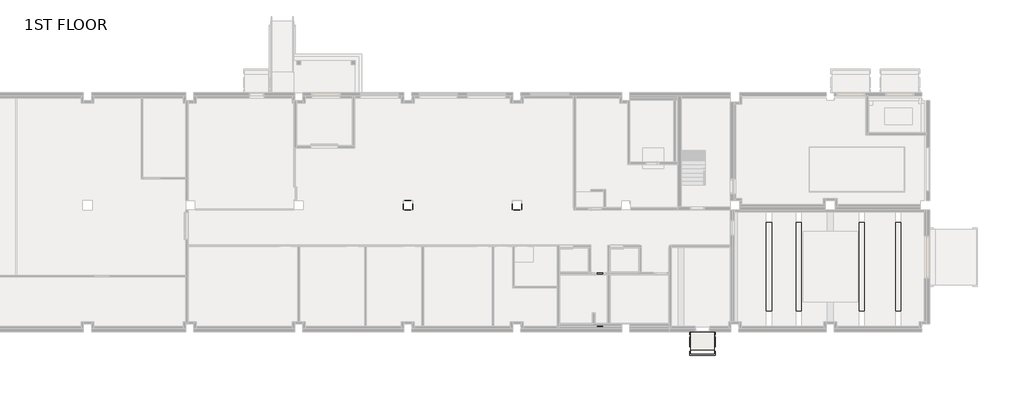
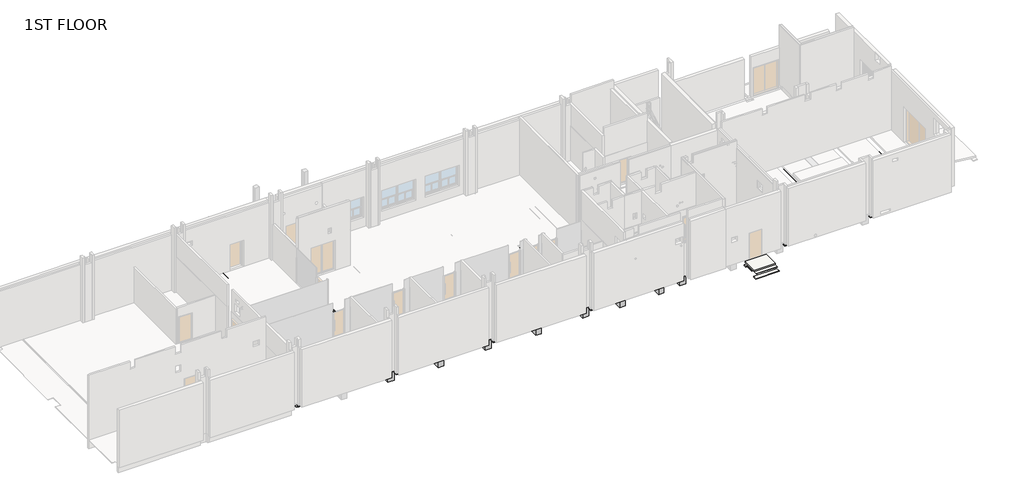
# One storey, part 9 of 15: 19 beams, 7 slabs.
"""IFC4 building model written with IfcOpenShell, lengths in millimetres."""

from ifc_helpers import new_model, si_unit, frame, origin, place, context, project, spatial, polyline, outline, extrude, faceted_brep, element, save

model = new_model("IFC4")

# Units and contexts
model_context = context("Model", 3, world=origin())
ifc_project = project(units=[si_unit("LENGTHUNIT", "METRE", prefix="MILLI")], contexts=[model_context])

# Site, building, storey
site = spatial("IfcSite", under=ifc_project)
building = spatial("IfcBuilding", under=site)
storey = spatial("IfcBuildingStorey", under=building, Name="1ST FLOOR", Elevation=4800.0)

# Beams
placement = place(None, origin())
element("IfcBeam", 1, ObjectType="RC Beam_Rectangular : H_SB_AR S16_TG-UG_500x800_1G2", at=placement, inside=storey, context=model_context, shape_type="Brep", body=[
    faceted_brep([(22650.0, -8350.0, 4800.0), (22650.0, -7850.0, 4800.0), (19225.0, -7850.0, 4800.0), (18775.0, -7850.0, 4800.0), (15400.0000001, -7850.0, 4800.0), (15400.0000001, -8350.0, 4800.0), (18775.0, -8350.0, 4800.0), (19225.0, -8350.0, 4800.0), (22650.0, -7850.0, 4000.0), (19225.0, -7850.0, 4000.0), (18775.0, -7850.0, 4000.0), (15400.0000001, -7850.0, 4000.0), (15400.0000001, -7850.0, 4650.0), (22650.0, -7850.0, 4650.0), (22650.0, -8350.0, 4000.0), (19225.0, -8350.0, 4000.0), (18775.0, -8350.0, 4000.0), (15400.0000001, -8350.0, 4000.0), (22650.0, -8350.0, 4650.0), (15400.0000001, -8350.0, 4650.0)], [[[0, 1, 2, 3, 4, 5, 6, 7]], [[8, 9, 10, 11, 12, 4, 3, 2, 1, 13]], [[11, 10, 9, 8, 14, 15, 16, 17]], [[17, 16, 15, 14, 18, 0, 7, 6, 5, 19]], [[14, 8, 13, 1, 0, 18]], [[5, 4, 12, 11, 17, 19]]]),
])
element("IfcBeam", 2, ObjectType="RC Beam_Rectangular : H_SB_AR S16_TG-UG_500x800_1G2", at=placement, inside=storey, context=model_context, shape_type="Brep", body=[
    faceted_brep([(23350.0, -7850.0, 4800.0), (23350.0, -8350.0, 4800.0), (26775.0, -8350.0, 4800.0), (27225.0, -8350.0, 4800.0), (30650.0, -8350.0, 4800.0), (30650.0, -7850.0, 4800.0), (27225.0, -7850.0, 4800.0), (26775.0, -7850.0, 4800.0), (23350.0, -8350.0, 4000.0), (26775.0, -8350.0, 4000.0), (27225.0, -8350.0, 4000.0), (30650.0, -8350.0, 4000.0), (30650.0, -8350.0, 4650.0), (23350.0, -8350.0, 4650.0), (23350.0, -7850.0, 4000.0), (26775.0, -7850.0, 4000.0), (27225.0, -7850.0, 4000.0), (30650.0, -7850.0, 4000.0), (23350.0, -7850.0, 4650.0), (30650.0, -7850.0, 4650.0)], [[[0, 1, 2, 3, 4, 5, 6, 7]], [[8, 9, 10, 11, 12, 4, 3, 2, 1, 13]], [[11, 10, 9, 8, 14, 15, 16, 17]], [[17, 16, 15, 14, 18, 0, 7, 6, 5, 19]], [[14, 8, 13, 1, 0, 18]], [[5, 4, 12, 11, 17, 19]]]),
])
element("IfcBeam", 3, ObjectType="RC Beam_Rectangular : H_SB_AR S16_TG-UG_500x800_1G2", at=placement, inside=storey, context=model_context, shape_type="Brep", body=[
    faceted_brep([(31350.0, -7850.0, 4800.0), (31350.0, -8350.0, 4800.0), (34775.0, -8350.0, 4800.0), (35225.0, -8350.0, 4800.0), (38650.0, -8350.0, 4800.0), (38650.0, -7850.0, 4800.0), (35225.0, -7850.0, 4800.0), (34775.0, -7850.0, 4800.0), (31350.0, -8350.0, 4000.0), (34775.0, -8350.0, 4000.0), (35225.0, -8350.0, 4000.0), (38650.0, -8350.0, 4000.0), (38650.0, -8350.0, 4650.0), (31350.0, -8350.0, 4650.0), (31350.0, -7850.0, 4000.0), (34775.0, -7850.0, 4000.0), (35225.0, -7850.0, 4000.0), (38650.0, -7850.0, 4000.0), (31350.0, -7850.0, 4650.0), (38650.0, -7850.0, 4650.0)], [[[0, 1, 2, 3, 4, 5, 6, 7]], [[8, 9, 10, 11, 12, 4, 3, 2, 1, 13]], [[11, 10, 9, 8, 14, 15, 16, 17]], [[17, 16, 15, 14, 18, 0, 7, 6, 5, 19]], [[14, 8, 13, 1, 0, 18]], [[5, 4, 12, 11, 17, 19]]]),
])
element("IfcBeam", 4, ObjectType="RC Beam_Rectangular : H_SB_AR S16_TG-UG_500x800_1G2", at=placement, inside=storey, context=model_context, shape_type="Brep", body=[
    faceted_brep([(39350.0, -7850.0, 4800.0), (39350.0, -8350.0, 4800.0), (41675.0, -8350.0, 4800.0), (42125.0, -8350.0, 4800.0), (44875.0, -8350.0, 4800.0), (45325.0, -8350.0, 4800.0), (46650.0, -8350.0, 4800.0), (46650.0, -7850.0, 4800.0), (45325.0, -7850.0, 4800.0), (44875.0, -7850.0, 4800.0), (42125.0, -7850.0, 4800.0), (41675.0, -7850.0, 4800.0), (39350.0, -8350.0, 4000.0), (41675.0, -8350.0, 4000.0), (42125.0, -8350.0, 4000.0), (44875.0, -8350.0, 4000.0), (45325.0, -8350.0, 4000.0), (46650.0, -8350.0, 4000.0), (46650.0, -8350.0, 4650.0), (39350.0, -8350.0, 4650.0), (39350.0, -7850.0, 4000.0), (41675.0, -7850.0, 4000.0), (42125.0, -7850.0, 4000.0), (44875.0, -7850.0, 4000.0), (45325.0, -7850.0, 4000.0), (46650.0, -7850.0, 4000.0), (39350.0, -7850.0, 4650.0), (46650.0, -7850.0, 4650.0)], [[[0, 1, 2, 3, 4, 5, 6, 7, 8, 9, 10, 11]], [[12, 13, 14, 15, 16, 17, 18, 6, 5, 4, 3, 2, 1, 19]], [[17, 16, 15, 14, 13, 12, 20, 21, 22, 23, 24, 25]], [[25, 24, 23, 22, 21, 20, 26, 0, 11, 10, 9, 8, 7, 27]], [[20, 12, 19, 1, 0, 26]], [[7, 6, 18, 17, 25, 27]]]),
])
element("IfcBeam", 5, ObjectType="RC Beam_Rectangular : H_SB_AR S16_TG-UG_500x800_1G1", at=placement, inside=storey, context=model_context, shape_type="Brep", body=[
    faceted_brep([(22700.0, -300.0, 4800.0), (22700.0, -7650.0, 4800.0), (23200.0, -7650.0, 4800.0), (23200.0, -300.0, 4800.0), (23200.0, -7650.0, 4650.0), (23200.0, -7650.0, 4000.0), (23200.0, -300.0, 4000.0), (23200.0, -300.0, 4650.0), (22700.0, -7650.0, 4000.0), (22700.0, -300.0, 4000.0), (22700.0, -300.0, 4650.0), (22700.0, -7650.0, 4650.0)], [[[0, 1, 2, 3]], [[3, 2, 4, 5, 6, 7]], [[6, 5, 8, 9]], [[1, 0, 10, 9, 8, 11]], [[8, 5, 4, 2, 1, 11]], [[0, 3, 7, 6, 9, 10]]]),
])
element("IfcBeam", 6, ObjectType="RC Beam_Rectangular : H_SB_AR S16_TG-UG_450x800_1B1", at=placement, inside=storey, context=model_context, shape_type="Brep", body=[
    faceted_brep([(19225.0, -100.0, 4800.0), (18775.0, -100.0, 4800.0), (18775.0, -7850.0, 4800.0), (19225.0, -7850.0, 4800.0), (19225.0, -7850.0, 4650.0), (19225.0, -7850.0, 4000.0), (19225.0, -100.0, 4000.0), (19225.0, -100.0, 4650.0), (18775.0, -100.0, 4000.0), (18775.0, -7850.0, 4000.0), (18775.0, -100.0, 4650.0), (18775.0, -7850.0, 4650.0)], [[[0, 1, 2, 3]], [[0, 3, 4, 5, 6, 7]], [[8, 6, 5, 9]], [[2, 1, 10, 8, 9, 11]], [[1, 0, 7, 6, 8, 10]], [[3, 2, 11, 9, 5, 4]]]),
])
element("IfcBeam", 7, ObjectType="RC Beam_Rectangular : H_SB_AR S16_TG-UG_500x800_1G1", at=placement, inside=storey, context=model_context, shape_type="Brep", body=[
    faceted_brep([(30750.0, -300.0, 4800.0), (30750.0, -7650.0, 4800.0), (31250.0, -7650.0, 4800.0), (31250.0, -300.0, 4800.0), (31250.0, -7650.0, 4650.0), (31250.0, -7650.0, 4000.0), (31250.0, -300.0, 4000.0), (31250.0, -300.0, 4650.0), (30750.0, -7650.0, 4000.0), (30750.0, -300.0, 4000.0), (30750.0, -300.0, 4650.0), (30750.0, -7650.0, 4650.0)], [[[0, 1, 2, 3]], [[3, 2, 4, 5, 6, 7]], [[6, 5, 8, 9]], [[1, 0, 10, 9, 8, 11]], [[8, 5, 4, 2, 1, 11]], [[0, 3, 7, 6, 9, 10]]]),
])
element("IfcBeam", 8, ObjectType="RC Beam_Rectangular : H_SB_AR S16_TG-UG_450x800_1B1", at=placement, inside=storey, context=model_context, shape_type="Brep", body=[
    faceted_brep([(27225.0, -100.0, 4800.0), (26775.0, -100.0, 4800.0), (26775.0, -7850.0, 4800.0), (27225.0, -7850.0, 4800.0), (27225.0, -7850.0, 4650.0), (27225.0, -7850.0, 4000.0), (27225.0, -100.0, 4000.0), (27225.0, -100.0, 4650.0), (26775.0, -100.0, 4000.0), (26775.0, -7850.0, 4000.0), (26775.0, -100.0, 4650.0), (26775.0, -7850.0, 4650.0)], [[[0, 1, 2, 3]], [[0, 3, 4, 5, 6, 7]], [[8, 6, 5, 9]], [[2, 1, 10, 8, 9, 11]], [[1, 0, 7, 6, 8, 10]], [[3, 2, 11, 9, 5, 4]]]),
])
element("IfcBeam", 9, ObjectType="RC Beam_Rectangular : H_SB_AR S16_TG-UG_450x800_1B1", at=placement, inside=storey, context=model_context, shape_type="Brep", body=[
    faceted_brep([(35225.0, -100.0, 4800.0), (34775.0, -100.0, 4800.0), (34775.0, -7850.0, 4800.0), (35225.0, -7850.0, 4800.0), (35225.0, -7850.0, 4650.0), (35225.0, -7850.0, 4000.0), (35225.0, -100.0, 4000.0), (35225.0, -100.0, 4650.0), (34775.0, -100.0, 4000.0), (34775.0, -7850.0, 4000.0), (34775.0, -100.0, 4650.0), (34775.0, -7850.0, 4650.0)], [[[0, 1, 2, 3]], [[0, 3, 4, 5, 6, 7]], [[8, 6, 5, 9]], [[2, 1, 10, 8, 9, 11]], [[1, 0, 7, 6, 8, 10]], [[3, 2, 11, 9, 5, 4]]]),
])
element("IfcBeam", 10, ObjectType="RC Beam_Rectangular : H_SB_AR S16_TG-UG_500x800_1G1", at=placement, inside=storey, context=model_context, shape_type="Brep", body=[
    faceted_brep([(22750.0, -8350.0, 4800.0), (22750.0, -16700.0, 4800.0), (23250.0, -16700.0, 4800.0), (23250.0, -8350.0, 4800.0), (23250.0, -16700.0, 4650.0), (23250.0, -16700.0, 4000.0), (23250.0, -8350.0, 4000.0), (23250.0, -8350.0, 4650.0), (22750.0, -16700.0, 4000.0), (22750.0, -8350.0, 4000.0), (22750.0, -8350.0, 4650.0), (22750.0, -16700.0, 4650.0)], [[[0, 1, 2, 3]], [[3, 2, 4, 5, 6, 7]], [[6, 5, 8, 9]], [[1, 0, 10, 9, 8, 11]], [[0, 3, 7, 6, 9, 10]], [[8, 5, 4, 2, 1, 11]]]),
])
element("IfcBeam", 11, ObjectType="RC Beam_Rectangular : H_SB_AR S16_TG-UG_500x800_1G1", at=placement, inside=storey, context=model_context, shape_type="Brep", body=[
    faceted_brep([(30750.0, -8350.0, 4800.0), (30750.0, -16700.0, 4800.0), (31250.0, -16700.0, 4800.0), (31250.0, -8350.0, 4800.0), (31250.0, -16700.0, 4650.0), (31250.0, -16700.0, 4000.0), (31250.0, -8350.0, 4000.0), (31250.0, -8350.0, 4650.0), (30750.0, -16700.0, 4000.0), (30750.0, -8350.0, 4000.0), (30750.0, -8350.0, 4650.0), (30750.0, -16700.0, 4650.0)], [[[0, 1, 2, 3]], [[3, 2, 4, 5, 6, 7]], [[6, 5, 8, 9]], [[1, 0, 10, 9, 8, 11]], [[0, 3, 7, 6, 9, 10]], [[8, 5, 4, 2, 1, 11]]]),
])
element("IfcBeam", 12, ObjectType="RC Beam_Rectangular : H_SB_AR S16_TG-UG_500x800_1G1", at=placement, inside=storey, context=model_context, shape_type="Brep", body=[
    faceted_brep([(38750.0000001, -8350.0, 4800.0), (38750.0000001, -16700.0, 4800.0), (39250.0000001, -16700.0, 4800.0), (39250.0000001, -8350.0, 4800.0), (39250.0000001, -16700.0, 4650.0), (39250.0000001, -16700.0, 4000.0), (39250.0000001, -8350.0, 4000.0), (39250.0000001, -8350.0, 4650.0), (38750.0000001, -16700.0, 4000.0), (38750.0000001, -8350.0, 4000.0), (38750.0000001, -8350.0, 4650.0), (38750.0000001, -16700.0, 4650.0)], [[[0, 1, 2, 3]], [[3, 2, 4, 5, 6, 7]], [[6, 5, 8, 9]], [[1, 0, 10, 9, 8, 11]], [[0, 3, 7, 6, 9, 10]], [[8, 5, 4, 2, 1, 11]]]),
])
element("IfcBeam", 13, ObjectType="RC Beam_Rectangular : H_SB_AR S16_TG-UG_450x800_1B1A", at=placement, inside=storey, context=model_context, shape_type="Brep", body=[
    faceted_brep([(26775.0, -16900.0, 4800.0), (27225.0, -16900.0, 4800.0), (27225.0, -8350.0, 4800.0), (26775.0, -8350.0, 4800.0), (27225.0, -16900.0, 4650.0), (27225.0, -16900.0, 4000.0), (27225.0, -8350.0, 4000.0), (27225.0, -8350.0, 4650.0), (26775.0, -16900.0, 4000.0), (26775.0, -8350.0, 4000.0), (26775.0, -8350.0, 4650.0), (26775.0, -16900.0, 4650.0)], [[[0, 1, 2, 3]], [[2, 1, 4, 5, 6, 7]], [[5, 8, 9, 6]], [[0, 3, 10, 9, 8, 11]], [[1, 0, 11, 8, 5, 4]], [[3, 2, 7, 6, 9, 10]]]),
])
element("IfcBeam", 14, ObjectType="RC Beam_Rectangular : H_SB_AR S16_TG-UG_450x800_1B1A", at=placement, inside=storey, context=model_context, shape_type="Brep", body=[
    faceted_brep([(34775.0, -16900.0, 4800.0), (35225.0, -16900.0, 4800.0), (35225.0, -8350.0, 4800.0), (34775.0, -8350.0, 4800.0), (35225.0, -16900.0, 4650.0), (35225.0, -16900.0, 4000.0), (35225.0, -8350.0, 4000.0), (35225.0, -8350.0, 4650.0), (34775.0, -16900.0, 4000.0), (34775.0, -8350.0, 4000.0), (34775.0, -8350.0, 4650.0), (34775.0, -16900.0, 4650.0)], [[[0, 1, 2, 3]], [[2, 1, 4, 5, 6, 7]], [[5, 8, 9, 6]], [[0, 3, 10, 9, 8, 11]], [[1, 0, 11, 8, 5, 4]], [[3, 2, 7, 6, 9, 10]]]),
])
element("IfcBeam", 15, ObjectType="RC Beam_Rectangular : H_SB_AR S16_TG-UG_450x800_1B1A", at=placement, inside=storey, context=model_context, shape_type="Brep", body=[
    faceted_brep([(42125.0, -8350.0, 4800.0), (41675.0, -8350.0, 4800.0), (41675.0, -16900.0, 4800.0), (42125.0, -16900.0, 4800.0), (42125.0, -11075.0, 4800.0), (42125.0, -16900.0, 4700.0), (42125.0, -16900.0, 4550.0), (42125.0, -16900.0, 4000.0), (42125.0, -8350.0, 4000.0), (42125.0, -8350.0, 4650.0), (41675.0, -16900.0, 4000.0), (41675.0, -8350.0, 4000.0), (41675.0, -16900.0, 4650.0), (41675.0, -8350.0, 4650.0)], [[[0, 1, 2, 3, 4]], [[3, 5, 6, 7, 8, 9, 0, 4]], [[7, 10, 11, 8]], [[11, 10, 12, 2, 1, 13]], [[7, 6, 5, 3, 2, 12, 10]], [[1, 0, 9, 8, 11, 13]]]),
])
element("IfcBeam", 16, ObjectType="RC Beam_Rectangular : H_SB_AR S16_TG-UG_450x700_1B1B", at=placement, inside=storey, context=model_context, shape_type="Brep", body=[
    faceted_brep([(44875.0, -13075.0, 4700.0), (45325.0, -13075.0, 4700.0), (45325.0, -13075.0, 4650.0), (45325.0, -13075.0, 4550.0), (45325.0, -13075.0, 4000.0), (44875.0, -13075.0, 4000.0), (44875.0, -13075.0, 4550.0), (44875.0, -13075.0, 4650.0), (44875.0, -16900.0, 4700.0), (45325.0, -16900.0, 4700.0), (45325.0, -16900.0, 4550.0), (45325.0, -16900.0, 4000.0), (44875.0, -16900.0, 4000.0), (44875.0, -16900.0, 4550.0)], [[[0, 1, 2, 3, 4, 5, 6, 7]], [[1, 0, 8, 9]], [[1, 9, 10, 11, 4, 3, 2]], [[5, 4, 11, 12]], [[8, 0, 7, 6, 5, 12, 13]], [[12, 11, 10, 9, 8, 13]]]),
])
element("IfcBeam", 17, ObjectType="RC Beam_Rectangular : H_SB_AR S16_TG-UG_500x700_1G1A", at=placement, inside=storey, context=model_context, shape_type="Brep", body=[
    faceted_brep([(46750.0, -11075.0, 4700.0), (47250.0, -11075.0, 4700.0), (47250.0, -11075.0, 4550.0), (47250.0, -11075.0, 4000.0), (46750.0, -11075.0, 4000.0), (46750.0, -11075.0, 4550.0), (46750.0, -16700.0, 4700.0), (47250.0, -16700.0, 4700.0), (47250.0, -16700.0, 4550.0), (47250.0, -16700.0, 4000.0), (46750.0, -16700.0, 4000.0), (46750.0, -16700.0, 4550.0)], [[[0, 1, 2, 3, 4, 5]], [[1, 0, 6, 7]], [[1, 7, 8, 9, 3, 2]], [[4, 3, 9, 10]], [[6, 0, 5, 4, 10, 11]], [[10, 9, 8, 7, 6, 11]]]),
])
element("IfcBeam", 18, ObjectType="RC Beam_Rectangular : H_SB_AR S16_TG-UG_500x800_1G1A", at=placement, inside=storey, context=model_context, shape_type="Brep", body=[
    faceted_brep([(46750.0, -11075.0, 4000.0), (47250.0, -11075.0, 4000.0), (47250.0, -11075.0, 4650.0), (47250.0, -11075.0, 4700.0), (47250.0, -11075.0, 4800.0), (46750.0, -11075.0, 4800.0), (46750.0, -11075.0, 4700.0), (46750.0, -11075.0, 4650.0), (47250.0, -8350.0, 4800.0), (46750.0, -8350.0, 4800.0), (47250.0, -8350.0, 4000.0), (47250.0, -8350.0, 4650.0), (46750.0, -8350.0, 4000.0), (46750.0, -8350.0, 4650.0)], [[[0, 1, 2, 3, 4, 5, 6, 7]], [[5, 4, 8, 9]], [[8, 4, 3, 2, 1, 10, 11]], [[1, 0, 12, 10]], [[5, 9, 13, 12, 0, 7, 6]], [[9, 8, 11, 10, 12, 13]]]),
])
element("IfcBeam", 19, ObjectType="RC Beam_Rectangular : H_SB_AR S16_TG-UG_450x800_1B1B", at=placement, inside=storey, context=model_context, shape_type="Brep", body=[
    faceted_brep([(44875.0, -13075.0, 4000.0), (45325.0, -13075.0, 4000.0), (45325.0, -13075.0, 4650.0), (45325.0, -13075.0, 4700.0), (45325.0, -13075.0, 4800.0), (44875.0, -13075.0, 4800.0), (44875.0, -13075.0, 4700.0), (44875.0, -13075.0, 4650.0), (45325.0, -8350.0, 4800.0), (44875.0, -8350.0, 4800.0), (45325.0, -8350.0, 4000.0), (45325.0, -8350.0, 4650.0), (44875.0, -8350.0, 4000.0), (44875.0, -8350.0, 4650.0)], [[[0, 1, 2, 3, 4, 5, 6, 7]], [[5, 4, 8, 9]], [[8, 4, 3, 2, 1, 10, 11]], [[1, 0, 12, 10]], [[5, 9, 13, 12, 0, 7, 6]], [[9, 8, 11, 10, 12, 13]]]),
])

# Slabs
element("IfcSlab", 20, ObjectType="H_SF_AR_B08_Stoop_T150", at=placement, inside=storey, context=model_context, shape_type="Brep", body=[
    faceted_brep([(51775.0, -18599.9999926, 4600.0), (51775.0, -18399.9999926, 4600.0), (51775.0, -17662.0, 4600.0), (51775.0, -17312.0, 4600.0), (53475.0, -17312.0, 4600.0), (53475.0, -17662.0, 4600.0), (53475.0, -18399.9999926, 4600.0), (53475.0, -18599.9999926, 4600.0), (51775.0, -18599.9999926, 4750.0), (53475.0, -18599.9999926, 4750.0), (53475.0, -17312.0, 4750.0), (51775.0, -17312.0, 4750.0), (51775.0, -18599.9999926, 4625.0), (53475.0, -18599.9999926, 4625.0)], [[[0, 1, 2, 3, 4, 5, 6, 7]], [[8, 9, 10, 11]], [[3, 2, 1, 0, 12, 8, 11]], [[4, 3, 11, 10]], [[7, 6, 5, 4, 10, 9, 13]], [[0, 7, 13, 9, 8, 12]]]),
])
element("IfcSlab", 21, ObjectType="H_SF_AR_B08_Stoop_T125", at=placement, inside=storey, context=model_context, shape_type="SweptSolid", body=[
    extrude(outline(polyline([(51775.0, -18899.9999926), (51775.0, -18599.9999926), (53475.0, -18599.9999926), (53475.0, -18899.9999926), (51775.0, -18899.9999926)])), frame((0.0, 0.0, 4600.0), z_axis=(0.0, 0.0, 1.0), x_axis=(1.0, 0.0, 0.0)), (0.0, 0.0, 1.0), 25.0),
])
element("IfcSlab", 22, ObjectType="H_SF_AR_S18_Lean_T50", at=placement, inside=storey, context=model_context, shape_type="SweptSolid", body=[
    extrude(outline(polyline([(51675.0, -18999.9999926), (51675.0, -18699.9999926), (53575.0, -18699.9999926), (53575.0, -18999.9999926), (51675.0, -18999.9999926)])), frame((0.0, 0.0, 4250.0), z_axis=(0.0, 0.0, 1.0), x_axis=(1.0, 0.0, 0.0)), (0.0, 0.0, 1.0), 50.0),
])
element("IfcSlab", 23, ObjectType="H_SF_AR_S18_Lean_T50", at=placement, inside=storey, context=model_context, shape_type="SweptSolid", body=[
    extrude(outline(polyline([(51675.0, -17299.9999926), (53575.0, -17299.9999926), (53575.0, -17512.0), (51675.0, -17512.0), (51675.0, -17299.9999926)])), frame((0.0, 0.0, 4400.0), z_axis=(0.0, 0.0, 1.0), x_axis=(1.0, 0.0, 0.0)), (0.0, 0.0, 1.0), 50.0),
])
element("IfcSlab", 24, ObjectType="H_SF_AR_S18_Lean_T50", at=placement, inside=storey, context=model_context, shape_type="Brep", body=[
    faceted_brep([(51675.0, -18399.9999926, 4550.0), (51675.0, -18379.2893145, 4550.0), (51675.0, -17682.7106781, 4550.0), (51675.0, -17662.0, 4550.0), (53575.0, -17662.0, 4550.0), (53575.0, -17682.7106781, 4550.0), (53575.0, -18379.2893145, 4550.0), (53575.0, -18399.9999926, 4550.0), (51675.0, -18399.9999926, 4600.0), (53575.0, -18399.9999926, 4600.0), (53575.0, -17662.0, 4600.0), (51675.0, -17662.0, 4600.0)], [[[0, 1, 2, 3, 4, 5, 6, 7]], [[8, 9, 10, 11]], [[3, 2, 1, 0, 8, 11]], [[4, 3, 11, 10]], [[7, 6, 5, 4, 10, 9]], [[0, 7, 9, 8]]]),
])
element("IfcSlab", 25, ObjectType="H_SF_AR_S18_Lean_T50", at=placement, inside=storey, context=model_context, shape_type="Brep", body=[
    faceted_brep([(19435.0, -1250.0000001, 3840.0), (19435.0, -7640.0, 3840.0), (21750.0000003, -7640.0, 3840.0), (21750.0000003, -8560.0, 3840.0), (19435.0, -8560.0, 3840.0), (19435.0, -15750.0000001, 3840.0), (18565.0, -15750.0000001, 3840.0), (18565.0, -8560.0, 3840.0), (16300.0000001, -8560.0, 3840.0), (16300.0000001, -7640.0, 3840.0), (18565.0, -7640.0, 3840.0), (18565.0, -1250.0000001, 3840.0), (19435.0, -7640.0, 3890.0), (19435.0, -1250.0000001, 3890.0), (18565.0, -1250.0000001, 3890.0), (18565.0, -7640.0, 3890.0), (16300.0000001, -7640.0, 3890.0), (16300.0000001, -8560.0, 3890.0), (18565.0, -8560.0, 3890.0), (18565.0, -15750.0000001, 3890.0), (19435.0, -15750.0000001, 3890.0), (19435.0, -8560.0, 3890.0), (21750.0000003, -8560.0, 3890.0), (21750.0000003, -7640.0, 3890.0)], [[[0, 1, 2, 3, 4, 5, 6, 7, 8, 9, 10, 11]], [[12, 13, 14, 15, 16, 17, 18, 19, 20, 21, 22, 23]], [[1, 0, 13, 12]], [[2, 1, 12, 23]], [[3, 2, 23, 22]], [[4, 3, 22, 21]], [[5, 4, 21, 20]], [[7, 6, 19, 18]], [[8, 7, 18, 17]], [[9, 8, 17, 16]], [[10, 9, 16, 15]], [[11, 10, 15, 14]], [[0, 11, 14, 13]], [[6, 5, 20, 19]]]),
    faceted_brep([(23410.0, -1250.0000001, 3840.0), (23410.0, -6750.0, 3840.0), (22490.0, -6750.0, 3840.0), (22490.0, -1250.0000001, 3840.0), (23410.0, -6750.0, 3890.0), (23410.0, -1250.0000001, 3890.0), (22490.0, -1250.0000001, 3890.0), (22490.0, -6750.0, 3890.0)], [[[0, 1, 2, 3]], [[4, 5, 6, 7]], [[1, 0, 5, 4]], [[2, 1, 4, 7]], [[3, 2, 7, 6]], [[0, 3, 6, 5]]]),
    faceted_brep([(23460.0, -9250.0, 3840.0), (23460.0, -15750.0000001, 3840.0), (22540.0, -15750.0000001, 3840.0), (22540.0, -9250.0, 3840.0), (23460.0, -15750.0000001, 3890.0), (23460.0, -9250.0, 3890.0), (22540.0, -9250.0, 3890.0), (22540.0, -15750.0000001, 3890.0)], [[[0, 1, 2, 3]], [[4, 5, 6, 7]], [[1, 0, 5, 4]], [[2, 1, 4, 7]], [[3, 2, 7, 6]], [[0, 3, 6, 5]]]),
    faceted_brep([(27435.0, -1250.0000001, 3840.0), (27435.0, -7640.0, 3840.0), (29750.0000003, -7640.0, 3840.0), (29750.0000003, -8560.0, 3840.0), (27435.0, -8560.0, 3840.0), (27435.0, -15750.0000001, 3840.0), (26565.0, -15750.0000001, 3840.0), (26565.0, -8560.0, 3840.0), (24249.9999997, -8560.0, 3840.0), (24249.9999997, -7640.0, 3840.0), (26565.0, -7640.0, 3840.0), (26565.0, -1250.0000001, 3840.0), (27435.0, -7640.0, 3890.0), (27435.0, -1250.0000001, 3890.0), (26565.0, -1250.0000001, 3890.0), (26565.0, -7640.0, 3890.0), (24249.9999997, -7640.0, 3890.0), (24249.9999997, -8560.0, 3890.0), (26565.0, -8560.0, 3890.0), (26565.0, -15750.0000001, 3890.0), (27435.0, -15750.0000001, 3890.0), (27435.0, -8560.0, 3890.0), (29750.0000003, -8560.0, 3890.0), (29750.0000003, -7640.0, 3890.0)], [[[0, 1, 2, 3, 4, 5, 6, 7, 8, 9, 10, 11]], [[12, 13, 14, 15, 16, 17, 18, 19, 20, 21, 22, 23]], [[1, 0, 13, 12]], [[2, 1, 12, 23]], [[3, 2, 23, 22]], [[4, 3, 22, 21]], [[5, 4, 21, 20]], [[6, 5, 20, 19]], [[7, 6, 19, 18]], [[8, 7, 18, 17]], [[9, 8, 17, 16]], [[10, 9, 16, 15]], [[11, 10, 15, 14]], [[0, 11, 14, 13]]]),
    faceted_brep([(31459.9999999, -1250.0000001, 3840.0), (31459.9999999, -6750.0, 3840.0), (30539.9999999, -6750.0, 3840.0), (30539.9999999, -1250.0000001, 3840.0), (31459.9999999, -6750.0, 3890.0), (31459.9999999, -1250.0000001, 3890.0), (30539.9999999, -1250.0000001, 3890.0), (30539.9999999, -6750.0, 3890.0)], [[[0, 1, 2, 3]], [[4, 5, 6, 7]], [[1, 0, 5, 4]], [[2, 1, 4, 7]], [[3, 2, 7, 6]], [[0, 3, 6, 5]]]),
    faceted_brep([(31459.9999999, -9250.0, 3840.0), (31459.9999999, -15750.0000001, 3840.0), (30539.9999999, -15750.0000001, 3840.0), (30539.9999999, -9250.0, 3840.0), (31459.9999999, -15750.0000001, 3890.0), (31459.9999999, -9250.0, 3890.0), (30539.9999999, -9250.0, 3890.0), (30539.9999999, -15750.0000001, 3890.0)], [[[0, 1, 2, 3]], [[4, 5, 6, 7]], [[1, 0, 5, 4]], [[2, 1, 4, 7]], [[3, 2, 7, 6]], [[0, 3, 6, 5]]]),
    faceted_brep([(35435.0, -1250.0000001, 3840.0), (35435.0, -7640.0, 3840.0), (37750.0000003, -7640.0, 3840.0), (37750.0000003, -8560.0, 3840.0), (35435.0, -8560.0, 3840.0), (35435.0, -15750.0000001, 3840.0), (34565.0, -15750.0000001, 3840.0), (34565.0, -8560.0, 3840.0), (32250.0000002, -8560.0, 3840.0), (32250.0000002, -7640.0, 3840.0), (34565.0, -7640.0, 3840.0), (34565.0, -1250.0000001, 3840.0), (35435.0, -7640.0, 3890.0), (35435.0, -1250.0000001, 3890.0), (34565.0, -1250.0000001, 3890.0), (34565.0, -7640.0, 3890.0), (32250.0000002, -7640.0, 3890.0), (32250.0000002, -8560.0, 3890.0), (34565.0, -8560.0, 3890.0), (34565.0, -15750.0000001, 3890.0), (35435.0, -15750.0000001, 3890.0), (35435.0, -8560.0, 3890.0), (37750.0000003, -8560.0, 3890.0), (37750.0000003, -7640.0, 3890.0)], [[[0, 1, 2, 3, 4, 5, 6, 7, 8, 9, 10, 11]], [[12, 13, 14, 15, 16, 17, 18, 19, 20, 21, 22, 23]], [[1, 0, 13, 12]], [[2, 1, 12, 23]], [[3, 2, 23, 22]], [[4, 3, 22, 21]], [[5, 4, 21, 20]], [[6, 5, 20, 19]], [[7, 6, 19, 18]], [[8, 7, 18, 17]], [[9, 8, 17, 16]], [[10, 9, 16, 15]], [[11, 10, 15, 14]], [[0, 11, 14, 13]]]),
    faceted_brep([(39459.9999999, -1250.0000001, 3840.0), (39459.9999999, -6750.0, 3840.0), (38539.9999999, -6750.0, 3840.0), (38539.9999999, -1250.0000001, 3840.0), (39459.9999999, -6750.0, 3890.0), (39459.9999999, -1250.0000001, 3890.0), (38539.9999999, -1250.0000001, 3890.0), (38539.9999999, -6750.0, 3890.0)], [[[0, 1, 2, 3]], [[4, 5, 6, 7]], [[1, 0, 5, 4]], [[2, 1, 4, 7]], [[3, 2, 7, 6]], [[0, 3, 6, 5]]]),
    faceted_brep([(39459.9999999, -9250.0, 3840.0), (39459.9999999, -15750.0000001, 3840.0), (38539.9999999, -15750.0000001, 3840.0), (38539.9999999, -9250.0, 3840.0), (39459.9999999, -15750.0000001, 3890.0), (39459.9999999, -9250.0, 3890.0), (38539.9999999, -9250.0, 3890.0), (38539.9999999, -15750.0000001, 3890.0)], [[[0, 1, 2, 3]], [[4, 5, 6, 7]], [[1, 0, 5, 4]], [[2, 1, 4, 7]], [[3, 2, 7, 6]], [[0, 3, 6, 5]]]),
    faceted_brep([(42335.0, -1250.0000001, 3840.0), (42335.0, -7640.0, 3840.0), (44665.0, -7640.0, 3840.0), (44665.0, -1250.0000001, 3840.0), (45535.0, -1250.0000001, 3840.0), (45535.0, -7640.0, 3840.0), (45749.9999999, -7640.0, 3840.0), (45749.9999999, -8560.0, 3840.0), (45535.0, -8560.0, 3840.0), (45535.0, -15750.0000001, 3840.0), (44665.0, -15750.0000001, 3840.0), (44665.0, -8560.0, 3840.0), (42335.0, -8560.0, 3840.0), (42335.0, -15750.0000001, 3840.0), (41465.0, -15750.0000001, 3840.0), (41465.0, -8560.0, 3840.0), (40250.0000001, -8560.0, 3840.0), (40250.0000001, -7640.0, 3840.0), (41465.0, -7640.0, 3840.0), (41465.0, -1250.0000001, 3840.0), (42335.0, -7640.0, 3890.0), (42335.0, -1250.0000001, 3890.0), (41465.0, -1250.0000001, 3890.0), (41465.0, -7640.0, 3890.0), (40250.0000001, -7640.0, 3890.0), (40250.0000001, -8560.0, 3890.0), (41465.0, -8560.0, 3890.0), (41465.0, -15750.0000001, 3890.0), (42335.0, -15750.0000001, 3890.0), (42335.0, -8560.0, 3890.0), (44665.0, -8560.0, 3890.0), (44665.0, -15750.0000001, 3890.0), (45535.0, -15750.0000001, 3890.0), (45535.0, -8560.0, 3890.0), (45749.9999999, -8560.0, 3890.0), (45749.9999999, -7640.0, 3890.0), (45535.0, -7640.0, 3890.0), (45535.0, -1250.0000001, 3890.0), (44665.0, -1250.0000001, 3890.0), (44665.0, -7640.0, 3890.0)], [[[0, 1, 2, 3, 4, 5, 6, 7, 8, 9, 10, 11, 12, 13, 14, 15, 16, 17, 18, 19]], [[20, 21, 22, 23, 24, 25, 26, 27, 28, 29, 30, 31, 32, 33, 34, 35, 36, 37, 38, 39]], [[1, 0, 21, 20]], [[2, 1, 20, 39]], [[3, 2, 39, 38]], [[4, 3, 38, 37]], [[5, 4, 37, 36]], [[6, 5, 36, 35]], [[7, 6, 35, 34]], [[8, 7, 34, 33]], [[9, 8, 33, 32]], [[10, 9, 32, 31]], [[11, 10, 31, 30]], [[12, 11, 30, 29]], [[13, 12, 29, 28]], [[14, 13, 28, 27]], [[15, 14, 27, 26]], [[16, 15, 26, 25]], [[17, 16, 25, 24]], [[18, 17, 24, 23]], [[19, 18, 23, 22]], [[0, 19, 22, 21]]]),
    faceted_brep([(47509.9999996, -1250.0000001, 3840.0), (47509.9999996, -6750.0, 3840.0), (46589.9999996, -6750.0, 3840.0), (46589.9999996, -1250.0000001, 3840.0), (47509.9999996, -6750.0, 3890.0), (47509.9999996, -1250.0000001, 3890.0), (46589.9999996, -1250.0000001, 3890.0), (46589.9999996, -6750.0, 3890.0)], [[[0, 1, 2, 3]], [[4, 5, 6, 7]], [[1, 0, 5, 4]], [[2, 1, 4, 7]], [[3, 2, 7, 6]], [[0, 3, 6, 5]]]),
    faceted_brep([(47459.9999996, -9250.0, 3840.0), (47459.9999996, -15750.0000001, 3840.0), (47300.0, -15750.0000001, 3840.0), (46539.9999996, -15750.0000001, 3840.0), (46539.9999996, -9250.0, 3840.0), (47459.9999996, -15750.0000001, 3890.0), (47459.9999996, -9250.0, 3890.0), (46539.9999996, -9250.0, 3890.0), (46539.9999996, -15750.0000001, 3890.0), (47300.0, -15750.0000001, 3890.0)], [[[0, 1, 2, 3, 4]], [[5, 6, 7, 8, 9]], [[1, 0, 6, 5]], [[1, 5, 9, 8, 3, 2]], [[4, 3, 8, 7]], [[0, 4, 7, 6]]]),
    faceted_brep([(49700.0000002, -8560.0, 3840.0), (48249.9999999, -8560.0, 3840.0), (48249.9999999, -7640.0, 3840.0), (49700.0000002, -7640.0, 3840.0), (48249.9999999, -8560.0, 3890.0), (49700.0000002, -8560.0, 3890.0), (49700.0000002, -7640.0, 3890.0), (48249.9999999, -7640.0, 3890.0)], [[[0, 1, 2, 3]], [[4, 5, 6, 7]], [[1, 0, 5, 4]], [[2, 1, 4, 7]], [[3, 2, 7, 6]], [[0, 3, 6, 5]]]),
    faceted_brep([(50615.0, -15750.0000001, 3840.0), (50615.0, -9250.0, 3840.0), (51485.0, -9250.0, 3840.0), (51485.0, -15750.0000001, 3840.0), (50825.0, -15750.0000001, 3840.0), (50615.0, -9250.0, 3890.0), (50615.0, -15750.0000001, 3890.0), (50825.0, -15750.0000001, 3890.0), (51485.0, -15750.0000001, 3890.0), (51485.0, -9250.0, 3890.0)], [[[0, 1, 2, 3, 4]], [[5, 6, 7, 8, 9]], [[1, 0, 6, 5]], [[2, 1, 5, 9]], [[3, 2, 9, 8]], [[3, 8, 7, 6, 0, 4]]]),
    faceted_brep([(54490.0, -15750.0000001, 3840.0), (54490.0, -9250.0, 3840.0), (55410.0, -9250.0, 3840.0), (55410.0, -15750.0000001, 3840.0), (54490.0, -9250.0, 3890.0), (54490.0, -15750.0000001, 3890.0), (55410.0, -15750.0000001, 3890.0), (55410.0, -9250.0, 3890.0)], [[[0, 1, 2, 3]], [[4, 5, 6, 7]], [[1, 0, 5, 4]], [[2, 1, 4, 7]], [[3, 2, 7, 6]], [[0, 3, 6, 5]]]),
    faceted_brep([(57065.0, -15750.0000001, 3840.0), (57065.0, -9250.0, 3840.0), (57935.0, -9250.0, 3840.0), (57935.0, -15750.0000001, 3840.0), (57065.0, -9250.0, 3890.0), (57065.0, -15750.0000001, 3890.0), (57935.0, -15750.0000001, 3890.0), (57935.0, -9250.0, 3890.0)], [[[0, 1, 2, 3]], [[4, 5, 6, 7]], [[1, 0, 5, 4]], [[2, 1, 4, 7]], [[3, 2, 7, 6]], [[0, 3, 6, 5]]]),
    faceted_brep([(59265.0, -15750.0000001, 3840.0), (59265.0, -9250.0, 3840.0), (60135.0, -9250.0, 3840.0), (60135.0, -15750.0000001, 3840.0), (59265.0, -9250.0, 3890.0), (59265.0, -15750.0000001, 3890.0), (60135.0, -15750.0000001, 3890.0), (60135.0, -9250.0, 3890.0)], [[[0, 1, 2, 3]], [[4, 5, 6, 7]], [[1, 0, 5, 4]], [[2, 1, 4, 7]], [[3, 2, 7, 6]], [[0, 3, 6, 5]]]),
    faceted_brep([(61540.0, -15750.0000001, 3840.0), (61540.0, -9250.0, 3840.0), (62460.0, -9250.0, 3840.0), (62460.0, -15750.0000001, 3840.0), (61540.0, -9250.0, 3890.0), (61540.0, -15750.0000001, 3890.0), (62460.0, -15750.0000001, 3890.0), (62460.0, -9250.0, 3890.0)], [[[0, 1, 2, 3]], [[4, 5, 6, 7]], [[1, 0, 5, 4]], [[2, 1, 4, 7]], [[3, 2, 7, 6]], [[0, 3, 6, 5]]]),
    faceted_brep([(63865.0, -15750.0000001, 3840.0), (63865.0, -9250.0, 3840.0), (64735.0, -9250.0, 3840.0), (64735.0, -15750.0000001, 3840.0), (63865.0, -9250.0, 3890.0), (63865.0, -15750.0000001, 3890.0), (64735.0, -15750.0000001, 3890.0), (64735.0, -9250.0, 3890.0)], [[[0, 1, 2, 3]], [[4, 5, 6, 7]], [[1, 0, 5, 4]], [[2, 1, 4, 7]], [[3, 2, 7, 6]], [[0, 3, 6, 5]]]),
    faceted_brep([(66565.0, -15750.0000001, 3840.0), (66565.0, -9250.0, 3840.0), (67435.0, -9250.0, 3840.0), (67435.0, -15750.0000001, 3840.0), (66565.0, -9250.0, 3890.0), (66565.0, -15750.0000001, 3890.0), (67435.0, -15750.0000001, 3890.0), (67435.0, -9250.0, 3890.0)], [[[0, 1, 2, 3]], [[4, 5, 6, 7]], [[1, 0, 5, 4]], [[2, 1, 4, 7]], [[3, 2, 7, 6]], [[0, 3, 6, 5]]]),
])
element("IfcSlab", 26, ObjectType="H_SF_AR_S18_Lean_T50", at=placement, inside=storey, context=model_context, shape_type="Brep", body=[
    faceted_brep([(15210.0, -8460.0, 4490.0), (18665.0, -8460.0, 4490.0), (18665.0, -16790.0, 4490.0), (15300.0, -16790.0, 4490.0), (15300.0, -16700.0, 4490.0), (15210.0, -16700.0, 4490.0), (18665.0, -8460.0, 4540.0), (15210.0, -8460.0, 4540.0), (15210.0, -16700.0, 4540.0), (15300.0, -16700.0, 4540.0), (15300.0, -16790.0, 4540.0), (18665.0, -16790.0, 4540.0)], [[[0, 1, 2, 3, 4, 5]], [[6, 7, 8, 9, 10, 11]], [[1, 0, 7, 6]], [[2, 1, 6, 11]], [[3, 2, 11, 10]], [[4, 3, 10, 9]], [[5, 4, 9, 8]], [[0, 5, 8, 7]]]),
    faceted_brep([(15400.0000001, -7740.0, 4490.0), (15400.0000001, -7650.0, 4490.0), (15210.0, -7650.0, 4490.0), (15210.0, -300.0, 4490.0), (15300.0, -300.0, 4490.0), (15300.0, -210.0, 4490.0), (18665.0, -210.0, 4490.0), (18665.0, -7740.0, 4490.0), (15400.0000001, -7650.0, 4540.0), (15400.0000001, -7740.0, 4540.0), (18665.0, -7740.0, 4540.0), (18665.0, -210.0, 4540.0), (15300.0, -210.0, 4540.0), (15300.0, -300.0, 4540.0), (15210.0, -300.0, 4540.0), (15210.0, -7650.0, 4540.0)], [[[0, 1, 2, 3, 4, 5, 6, 7]], [[8, 9, 10, 11, 12, 13, 14, 15]], [[1, 0, 9, 8]], [[2, 1, 8, 15]], [[3, 2, 15, 14]], [[4, 3, 14, 13]], [[5, 4, 13, 12]], [[6, 5, 12, 11]], [[7, 6, 11, 10]], [[0, 7, 10, 9]]]),
    faceted_brep([(22640.0, -8460.0, 4490.0), (22640.0, -16790.0, 4490.0), (19335.0, -16790.0, 4490.0), (19335.0, -8460.0, 4490.0), (22640.0, -16790.0, 4540.0), (22640.0, -8460.0, 4540.0), (19335.0, -8460.0, 4540.0), (19335.0, -16790.0, 4540.0)], [[[0, 1, 2, 3]], [[4, 5, 6, 7]], [[1, 0, 5, 4]], [[2, 1, 4, 7]], [[3, 2, 7, 6]], [[0, 3, 6, 5]]]),
    faceted_brep([(22650.0000003, -7740.0, 4490.0), (19335.0, -7740.0, 4490.0), (19335.0, -210.0, 4490.0), (22590.0, -210.0, 4490.0), (22590.0, -7650.0, 4490.0), (22650.0000003, -7650.0, 4490.0), (19335.0, -7740.0, 4540.0), (22650.0000003, -7740.0, 4540.0), (22650.0000003, -7650.0, 4540.0), (22590.0, -7650.0, 4540.0), (22590.0, -210.0, 4540.0), (19335.0, -210.0, 4540.0)], [[[0, 1, 2, 3, 4, 5]], [[6, 7, 8, 9, 10, 11]], [[1, 0, 7, 6]], [[2, 1, 6, 11]], [[3, 2, 11, 10]], [[4, 3, 10, 9]], [[5, 4, 9, 8]], [[0, 5, 8, 7]]]),
    faceted_brep([(23360.0, -8460.0, 4490.0), (26665.0, -8460.0, 4490.0), (26665.0, -16790.0, 4490.0), (23360.0, -16790.0, 4490.0), (26665.0, -8460.0, 4540.0), (23360.0, -8460.0, 4540.0), (23360.0, -16790.0, 4540.0), (26665.0, -16790.0, 4540.0)], [[[0, 1, 2, 3]], [[4, 5, 6, 7]], [[1, 0, 5, 4]], [[2, 1, 4, 7]], [[3, 2, 7, 6]], [[0, 3, 6, 5]]]),
    faceted_brep([(23350.0000003, -7740.0, 4490.0), (23350.0000003, -7650.0, 4490.0), (23310.0, -7650.0, 4490.0), (23310.0, -210.0, 4490.0), (26665.0, -210.0, 4490.0), (26665.0, -7740.0, 4490.0), (23350.0000003, -7650.0, 4540.0), (23350.0000003, -7740.0, 4540.0), (26665.0, -7740.0, 4540.0), (26665.0, -210.0, 4540.0), (23310.0, -210.0, 4540.0), (23310.0, -7650.0, 4540.0)], [[[0, 1, 2, 3, 4, 5]], [[6, 7, 8, 9, 10, 11]], [[1, 0, 7, 6]], [[2, 1, 6, 11]], [[3, 2, 11, 10]], [[4, 3, 10, 9]], [[5, 4, 9, 8]], [[0, 5, 8, 7]]]),
    faceted_brep([(30640.0, -8460.0, 4490.0), (30640.0, -16790.0, 4490.0), (27335.0, -16790.0, 4490.0), (27335.0, -8460.0, 4490.0), (30640.0, -16790.0, 4540.0), (30640.0, -8460.0, 4540.0), (27335.0, -8460.0, 4540.0), (27335.0, -16790.0, 4540.0)], [[[0, 1, 2, 3]], [[4, 5, 6, 7]], [[1, 0, 5, 4]], [[2, 1, 4, 7]], [[3, 2, 7, 6]], [[0, 3, 6, 5]]]),
    faceted_brep([(30650.0000002, -7740.0, 4490.0), (27335.0, -7740.0, 4490.0), (27335.0, -210.0, 4490.0), (30640.0, -210.0, 4490.0), (30640.0, -7650.0, 4490.0), (30650.0000002, -7650.0, 4490.0), (27335.0, -7740.0, 4540.0), (30650.0000002, -7740.0, 4540.0), (30650.0000002, -7650.0, 4540.0), (30640.0, -7650.0, 4540.0), (30640.0, -210.0, 4540.0), (27335.0, -210.0, 4540.0)], [[[0, 1, 2, 3, 4, 5]], [[6, 7, 8, 9, 10, 11]], [[1, 0, 7, 6]], [[2, 1, 6, 11]], [[3, 2, 11, 10]], [[4, 3, 10, 9]], [[5, 4, 9, 8]], [[0, 5, 8, 7]]]),
    faceted_brep([(31360.0, -8460.0, 4490.0), (34665.0, -8460.0, 4490.0), (34665.0, -16790.0, 4490.0), (31360.0, -16790.0, 4490.0), (34665.0, -8460.0, 4540.0), (31360.0, -8460.0, 4540.0), (31360.0, -16790.0, 4540.0), (34665.0, -16790.0, 4540.0)], [[[0, 1, 2, 3]], [[4, 5, 6, 7]], [[1, 0, 5, 4]], [[2, 1, 4, 7]], [[3, 2, 7, 6]], [[0, 3, 6, 5]]]),
    faceted_brep([(31350.0000002, -7740.0, 4490.0), (31350.0000002, -7650.0, 4490.0), (31360.0, -7650.0, 4490.0), (31360.0, -210.0, 4490.0), (34665.0, -210.0, 4490.0), (34665.0, -7740.0, 4490.0), (31350.0000002, -7650.0, 4540.0), (31350.0000002, -7740.0, 4540.0), (34665.0, -7740.0, 4540.0), (34665.0, -210.0, 4540.0), (31360.0, -210.0, 4540.0), (31360.0, -7650.0, 4540.0)], [[[0, 1, 2, 3, 4, 5]], [[6, 7, 8, 9, 10, 11]], [[1, 0, 7, 6]], [[2, 1, 6, 11]], [[3, 2, 11, 10]], [[4, 3, 10, 9]], [[5, 4, 9, 8]], [[0, 5, 8, 7]]]),
    faceted_brep([(38640.0, -8460.0, 4490.0), (38640.0, -16790.0, 4490.0), (35335.0, -16790.0, 4490.0), (35335.0, -8460.0, 4490.0), (38640.0, -16790.0, 4540.0), (38640.0, -8460.0, 4540.0), (35335.0, -8460.0, 4540.0), (35335.0, -16790.0, 4540.0)], [[[0, 1, 2, 3]], [[4, 5, 6, 7]], [[1, 0, 5, 4]], [[2, 1, 4, 7]], [[3, 2, 7, 6]], [[0, 3, 6, 5]]]),
    faceted_brep([(38650.0000001, -7740.0, 4490.0), (35335.0, -7740.0, 4490.0), (35335.0, -210.0, 4490.0), (38640.0, -210.0, 4490.0), (38640.0, -7650.0, 4490.0), (38650.0000001, -7650.0, 4490.0), (35335.0, -7740.0, 4540.0), (38650.0000001, -7740.0, 4540.0), (38650.0000001, -7650.0, 4540.0), (38640.0, -7650.0, 4540.0), (38640.0, -210.0, 4540.0), (35335.0, -210.0, 4540.0)], [[[0, 1, 2, 3, 4, 5]], [[6, 7, 8, 9, 10, 11]], [[1, 0, 7, 6]], [[2, 1, 6, 11]], [[3, 2, 11, 10]], [[4, 3, 10, 9]], [[5, 4, 9, 8]], [[0, 5, 8, 7]]]),
    faceted_brep([(39360.0, -8460.0, 4490.0), (41565.0, -8460.0, 4490.0), (41565.0, -16790.0, 4490.0), (39360.0, -16790.0, 4490.0), (41565.0, -8460.0, 4540.0), (39360.0, -8460.0, 4540.0), (39360.0, -16790.0, 4540.0), (41565.0, -16790.0, 4540.0)], [[[0, 1, 2, 3]], [[4, 5, 6, 7]], [[1, 0, 5, 4]], [[2, 1, 4, 7]], [[3, 2, 7, 6]], [[0, 3, 6, 5]]]),
    faceted_brep([(39350.0000001, -7740.0, 4490.0), (39350.0000001, -7650.0, 4490.0), (39360.0, -7650.0, 4490.0), (39360.0, -210.0, 4490.0), (41565.0, -210.0, 4490.0), (41565.0, -7740.0, 4490.0), (39350.0000001, -7650.0, 4540.0), (39350.0000001, -7740.0, 4540.0), (41565.0, -7740.0, 4540.0), (41565.0, -210.0, 4540.0), (39360.0, -210.0, 4540.0), (39360.0, -7650.0, 4540.0)], [[[0, 1, 2, 3, 4, 5]], [[6, 7, 8, 9, 10, 11]], [[1, 0, 7, 6]], [[2, 1, 6, 11]], [[3, 2, 11, 10]], [[4, 3, 10, 9]], [[5, 4, 9, 8]], [[0, 5, 8, 7]]]),
    faceted_brep([(44765.0, -210.0, 4490.0), (44765.0, -7740.0, 4490.0), (42235.0, -7740.0, 4490.0), (42235.0, -210.0, 4490.0), (44765.0, -7740.0, 4540.0), (44765.0, -210.0, 4540.0), (42235.0, -210.0, 4540.0), (42235.0, -7740.0, 4540.0)], [[[0, 1, 2, 3]], [[4, 5, 6, 7]], [[1, 0, 5, 4]], [[2, 1, 4, 7]], [[3, 2, 7, 6]], [[0, 3, 6, 5]]]),
    faceted_brep([(45435.0, -8460.0, 4490.0), (46640.0, -8460.0, 4490.0), (46640.0, -10654.2893219, 4490.0), (46640.0, -10675.0, 4490.0), (45435.0, -10675.0, 4490.0), (45435.0, -10654.2893219, 4490.0), (45435.0, -8460.0, 4540.0), (45435.0, -10675.0, 4540.0), (46640.0, -10675.0, 4540.0), (46640.0, -8460.0, 4540.0)], [[[0, 1, 2, 3, 4, 5]], [[6, 7, 8, 9]], [[7, 6, 0, 5, 4]], [[1, 0, 6, 9]], [[9, 8, 3, 2, 1]], [[4, 3, 8, 7]]]),
    faceted_brep([(46700.0, -210.0, 4490.0), (46700.0, -300.0, 4490.0), (46690.0, -300.0, 4490.0), (46690.0, -7650.0, 4490.0), (46649.9999999, -7650.0, 4490.0), (46649.9999999, -7740.0, 4490.0), (45435.0, -7740.0, 4490.0), (45435.0, -210.0, 4490.0), (46700.0, -300.0, 4540.0), (46700.0, -210.0, 4540.0), (45435.0, -210.0, 4540.0), (45435.0, -7740.0, 4540.0), (46649.9999999, -7740.0, 4540.0), (46649.9999999, -7650.0, 4540.0), (46690.0, -7650.0, 4540.0), (46690.0, -300.0, 4540.0)], [[[0, 1, 2, 3, 4, 5, 6, 7]], [[8, 9, 10, 11, 12, 13, 14, 15]], [[1, 0, 9, 8]], [[2, 1, 8, 15]], [[3, 2, 15, 14]], [[4, 3, 14, 13]], [[5, 4, 13, 12]], [[6, 5, 12, 11]], [[7, 6, 11, 10]], [[0, 7, 10, 9]]]),
    faceted_brep([(50715.0, -4825.0, 4490.0), (50715.0, -7740.0, 4490.0), (47410.0, -7740.0, 4490.0), (47410.0, -4825.0, 4490.0), (50715.0, -7740.0, 4540.0), (50715.0, -4825.0, 4540.0), (47410.0, -4825.0, 4540.0), (47410.0, -7740.0, 4540.0)], [[[0, 1, 2, 3]], [[4, 5, 6, 7]], [[1, 0, 5, 4]], [[2, 1, 4, 7]], [[3, 2, 7, 6]], [[0, 3, 6, 5]]]),
    faceted_brep([(54590.0, -8460.0, 4490.0), (54590.0, -16790.0, 4490.0), (51385.0, -16790.0, 4490.0), (51385.0, -8460.0, 4490.0), (54590.0, -16790.0, 4540.0), (54590.0, -8460.0, 4540.0), (51385.0, -8460.0, 4540.0), (51385.0, -16790.0, 4540.0)], [[[0, 1, 2, 3]], [[4, 5, 6, 7]], [[1, 0, 5, 4]], [[2, 1, 4, 7]], [[3, 2, 7, 6]], [[0, 3, 6, 5]]]),
    faceted_brep([(57165.0, -16790.0, 4490.0), (55310.0, -16790.0, 4490.0), (55310.0, -8460.0, 4490.0), (57165.0, -8460.0, 4490.0), (55310.0, -16790.0, 4540.0), (57165.0, -16790.0, 4540.0), (57165.0, -8460.0, 4540.0), (55310.0, -8460.0, 4540.0)], [[[0, 1, 2, 3]], [[4, 5, 6, 7]], [[1, 0, 5, 4]], [[2, 1, 4, 7]], [[3, 2, 7, 6]], [[0, 3, 6, 5]]]),
    faceted_brep([(59365.0, -8460.0, 4490.0), (59365.0, -16790.0, 4490.0), (57835.0, -16790.0, 4490.0), (57835.0, -8460.0, 4490.0), (59365.0, -16790.0, 4540.0), (59365.0, -8460.0, 4540.0), (57835.0, -8460.0, 4540.0), (57835.0, -16790.0, 4540.0)], [[[0, 1, 2, 3]], [[4, 5, 6, 7]], [[1, 0, 5, 4]], [[2, 1, 4, 7]], [[3, 2, 7, 6]], [[0, 3, 6, 5]]]),
    faceted_brep([(61640.0, -16790.0, 4490.0), (60035.0, -16790.0, 4490.0), (60035.0, -8460.0, 4490.0), (61640.0, -8460.0, 4490.0), (60035.0, -16790.0, 4540.0), (61640.0, -16790.0, 4540.0), (61640.0, -8460.0, 4540.0), (60035.0, -8460.0, 4540.0)], [[[0, 1, 2, 3]], [[4, 5, 6, 7]], [[1, 0, 5, 4]], [[2, 1, 4, 7]], [[3, 2, 7, 6]], [[0, 3, 6, 5]]]),
    faceted_brep([(63965.0, -8460.0, 4490.0), (63965.0, -16790.0, 4490.0), (62360.0, -16790.0, 4490.0), (62360.0, -8460.0, 4490.0), (63965.0, -16790.0, 4540.0), (63965.0, -8460.0, 4540.0), (62360.0, -8460.0, 4540.0), (62360.0, -16790.0, 4540.0)], [[[0, 1, 2, 3]], [[4, 5, 6, 7]], [[1, 0, 5, 4]], [[2, 1, 4, 7]], [[3, 2, 7, 6]], [[0, 3, 6, 5]]]),
    faceted_brep([(66665.0, -8460.0, 4490.0), (66665.0, -16790.0, 4490.0), (64635.0, -16790.0, 4490.0), (64635.0, -8460.0, 4490.0), (66665.0, -16790.0, 4540.0), (66665.0, -8460.0, 4540.0), (64635.0, -8460.0, 4540.0), (64635.0, -16790.0, 4540.0)], [[[0, 1, 2, 3]], [[4, 5, 6, 7]], [[1, 0, 5, 4]], [[2, 1, 4, 7]], [[3, 2, 7, 6]], [[0, 3, 6, 5]]]),
    faceted_brep([(68700.0, -16790.0, 4490.0), (67335.0, -16790.0, 4490.0), (67335.0, -8460.0, 4490.0), (68790.0, -8460.0, 4490.0), (68790.0, -16700.0, 4490.0), (68700.0, -16700.0, 4490.0), (67335.0, -16790.0, 4540.0), (68700.0, -16790.0, 4540.0), (68700.0, -16700.0, 4540.0), (68790.0, -16700.0, 4540.0), (68790.0, -8460.0, 4540.0), (67335.0, -8460.0, 4540.0)], [[[0, 1, 2, 3, 4, 5]], [[6, 7, 8, 9, 10, 11]], [[1, 0, 7, 6]], [[2, 1, 6, 11]], [[3, 2, 11, 10]], [[4, 3, 10, 9]], [[5, 4, 9, 8]], [[0, 5, 8, 7]]]),
    faceted_brep([(50575.0, -16790.0, 4490.0), (50575.0, -12675.0, 4490.0), (48375.0, -12675.0, 4490.0), (48375.0, -10675.0, 4490.0), (47360.0, -10675.0, 4490.0), (47360.0, -10654.2893219, 4490.0), (47360.0, -8460.0, 4490.0), (50715.0, -8460.0, 4490.0), (50715.0, -16790.0, 4490.0), (50595.7106781, -16790.0, 4490.0), (50575.0, -12675.0, 4540.0), (50575.0, -16790.0, 4540.0), (50715.0, -16790.0, 4540.0), (50715.0, -8460.0, 4540.0), (47360.0, -8460.0, 4540.0), (47360.0, -10675.0, 4540.0), (48375.0, -10675.0, 4540.0), (48375.0, -12675.0, 4540.0)], [[[0, 1, 2, 3, 4, 5, 6, 7, 8, 9]], [[10, 11, 12, 13, 14, 15, 16, 17]], [[1, 0, 11, 10]], [[2, 1, 10, 17]], [[3, 2, 17, 16]], [[4, 3, 16, 15]], [[15, 14, 6, 5, 4]], [[7, 6, 14, 13]], [[8, 7, 13, 12]], [[12, 11, 0, 9, 8]]]),
    faceted_brep([(44765.0, -12675.0, 4490.0), (44675.0, -12675.0, 4490.0), (44675.0, -10675.0, 4490.0), (42235.0, -10675.0, 4490.0), (42235.0, -10654.2893219, 4490.0), (42235.0, -8460.0, 4490.0), (44765.0, -8460.0, 4490.0), (44765.0, -12654.2893219, 4490.0), (44765.0, -12675.0, 4540.0), (44765.0, -8460.0, 4540.0), (42235.0, -8460.0, 4540.0), (42235.0, -10675.0, 4540.0), (44675.0, -10675.0, 4540.0), (44675.0, -12675.0, 4540.0)], [[[0, 1, 2, 3, 4, 5, 6, 7]], [[8, 9, 10, 11, 12, 13]], [[9, 8, 0, 7, 6]], [[1, 0, 8, 13]], [[2, 1, 13, 12]], [[3, 2, 12, 11]], [[11, 10, 5, 4, 3]], [[6, 5, 10, 9]]]),
])

save(model, "model.ifc")

# Revit data of these elements
# Type "RC Beam_Rectangular : H_SB_AR S16_TG-UG_500x800_1G2"
#   Type Comments = "CV-UG"
#   중앙부 하부근 = ""
#   중앙부 상부근 = ""
#   중앙부 보조근 = ""
#   중앙부 늑근 = ""
#   외단부 하부근 = ""
#   외단부 상부근 = ""
#   외단부 보조근 = ""
#   외단부 늑근 = ""
#   부호 = "TG3"
#   내단부 하부근 = ""
#   내단부 상부근 = ""
#   내단부 보조근 = ""
#   내단부 늑근 = ""
#   ALL 하부근 = "3-D20"
#   ALL 상부근 = "3-D20"
#   ALL 보조근 = ""
#   ALL 늑근 = "2-D10 @120"
#   H_Rebar Ratio = 0.14
#   Width = 500 mm
#   Height = 800 mm
#   Length [instance default] = 1524 mm
#   b = 500 mm
#   h = 800 mm
#   hec_material3 [instance default] = none
#   hec_material2 [instance default] = none
#   hec_material1 [instance default] = none
#   Structural Material [instance default] = none
#   Assembly Code = ""
# Type "RC Beam_Rectangular : H_SB_AR S16_TG-UG_500x800_1G1"
#   Type Comments = "CV-UG"
#   중앙부 하부근 = ""
#   중앙부 상부근 = ""
#   중앙부 보조근 = ""
#   중앙부 늑근 = ""
#   외단부 하부근 = ""
#   외단부 상부근 = ""
#   외단부 보조근 = ""
#   외단부 늑근 = ""
#   부호 = "TG3"
#   내단부 하부근 = ""
#   내단부 상부근 = ""
#   내단부 보조근 = ""
#   내단부 늑근 = ""
#   ALL 하부근 = "3-D20"
#   ALL 상부근 = "3-D20"
#   ALL 보조근 = ""
#   ALL 늑근 = "2-D10 @120"
#   H_Rebar Ratio = 0.14
#   Width = 500 mm
#   Height = 800 mm
#   Length [instance default] = 1524 mm
#   b = 500 mm
#   h = 800 mm
#   hec_material3 [instance default] = none
#   hec_material2 [instance default] = none
#   hec_material1 [instance default] = none
#   Structural Material [instance default] = none
#   Assembly Code = ""
# Type "RC Beam_Rectangular : H_SB_AR S16_TG-UG_450x800_1B1"
#   Type Comments = "CV-UG"
#   중앙부 하부근 = ""
#   중앙부 상부근 = ""
#   중앙부 보조근 = ""
#   중앙부 늑근 = ""
#   외단부 하부근 = ""
#   외단부 상부근 = ""
#   외단부 보조근 = ""
#   외단부 늑근 = ""
#   부호 = "TG3"
#   내단부 하부근 = ""
#   내단부 상부근 = ""
#   내단부 보조근 = ""
#   내단부 늑근 = ""
#   ALL 하부근 = "3-D20"
#   ALL 상부근 = "3-D20"
#   ALL 보조근 = ""
#   ALL 늑근 = "2-D10 @120"
#   H_Rebar Ratio = 0.14
#   Width = 450 mm
#   Height = 800 mm
#   Length [instance default] = 1524 mm
#   b = 450 mm
#   h = 800 mm
#   hec_material3 [instance default] = none
#   hec_material2 [instance default] = none
#   hec_material1 [instance default] = none
#   Structural Material [instance default] = none
#   Assembly Code = ""
# Type "RC Beam_Rectangular : H_SB_AR S16_TG-UG_450x800_1B1A"
#   Type Comments = "CV-UG"
#   중앙부 하부근 = ""
#   중앙부 상부근 = ""
#   중앙부 보조근 = ""
#   중앙부 늑근 = ""
#   외단부 하부근 = ""
#   외단부 상부근 = ""
#   외단부 보조근 = ""
#   외단부 늑근 = ""
#   부호 = "TG3"
#   내단부 하부근 = ""
#   내단부 상부근 = ""
#   내단부 보조근 = ""
#   내단부 늑근 = ""
#   ALL 하부근 = "3-D20"
#   ALL 상부근 = "3-D20"
#   ALL 보조근 = ""
#   ALL 늑근 = "2-D10 @120"
#   H_Rebar Ratio = 0.14
#   Width = 450 mm
#   Height = 800 mm
#   Length [instance default] = 1524 mm
#   b = 450 mm
#   h = 800 mm
#   hec_material3 [instance default] = none
#   hec_material2 [instance default] = none
#   hec_material1 [instance default] = none
#   Structural Material [instance default] = none
#   Assembly Code = ""
# Type "RC Beam_Rectangular : H_SB_AR S16_TG-UG_450x700_1B1B"
#   Type Comments = "CV-UG"
#   중앙부 하부근 = ""
#   중앙부 상부근 = ""
#   중앙부 보조근 = ""
#   중앙부 늑근 = ""
#   외단부 하부근 = ""
#   외단부 상부근 = ""
#   외단부 보조근 = ""
#   외단부 늑근 = ""
#   부호 = "TG3"
#   내단부 하부근 = ""
#   내단부 상부근 = ""
#   내단부 보조근 = ""
#   내단부 늑근 = ""
#   ALL 하부근 = "3-D20"
#   ALL 상부근 = "3-D20"
#   ALL 보조근 = ""
#   ALL 늑근 = "2-D10 @120"
#   H_Rebar Ratio = 0.14
#   Width = 450 mm
#   Height = 700 mm
#   Length [instance default] = 1524 mm
#   b = 450 mm
#   h = 700 mm
#   hec_material3 [instance default] = none
#   hec_material2 [instance default] = none
#   hec_material1 [instance default] = none
#   Structural Material [instance default] = none
#   Assembly Code = ""
# Type "RC Beam_Rectangular : H_SB_AR S16_TG-UG_500x700_1G1A"
#   Type Comments = "CV-UG"
#   중앙부 하부근 = ""
#   중앙부 상부근 = ""
#   중앙부 보조근 = ""
#   중앙부 늑근 = ""
#   외단부 하부근 = ""
#   외단부 상부근 = ""
#   외단부 보조근 = ""
#   외단부 늑근 = ""
#   부호 = "TG3"
#   내단부 하부근 = ""
#   내단부 상부근 = ""
#   내단부 보조근 = ""
#   내단부 늑근 = ""
#   ALL 하부근 = "3-D20"
#   ALL 상부근 = "3-D20"
#   ALL 보조근 = ""
#   ALL 늑근 = "2-D10 @120"
#   H_Rebar Ratio = 0.14
#   Width = 500 mm
#   Height = 700 mm
#   Length [instance default] = 1524 mm
#   b = 500 mm
#   h = 700 mm
#   hec_material3 [instance default] = none
#   hec_material2 [instance default] = none
#   hec_material1 [instance default] = none
#   Structural Material [instance default] = none
#   Assembly Code = ""
# Type "RC Beam_Rectangular : H_SB_AR S16_TG-UG_500x800_1G1A"
#   Type Comments = "CV-UG"
#   중앙부 하부근 = ""
#   중앙부 상부근 = ""
#   중앙부 보조근 = ""
#   중앙부 늑근 = ""
#   외단부 하부근 = ""
#   외단부 상부근 = ""
#   외단부 보조근 = ""
#   외단부 늑근 = ""
#   부호 = "TG3"
#   내단부 하부근 = ""
#   내단부 상부근 = ""
#   내단부 보조근 = ""
#   내단부 늑근 = ""
#   ALL 하부근 = "3-D20"
#   ALL 상부근 = "3-D20"
#   ALL 보조근 = ""
#   ALL 늑근 = "2-D10 @120"
#   H_Rebar Ratio = 0.14
#   Width = 500 mm
#   Height = 800 mm
#   Length [instance default] = 1524 mm
#   b = 500 mm
#   h = 800 mm
#   hec_material3 [instance default] = none
#   hec_material2 [instance default] = none
#   hec_material1 [instance default] = none
#   Structural Material [instance default] = none
#   Assembly Code = ""
# Type "RC Beam_Rectangular : H_SB_AR S16_TG-UG_450x800_1B1B"
#   Type Comments = "CV-UG"
#   중앙부 하부근 = ""
#   중앙부 상부근 = ""
#   중앙부 보조근 = ""
